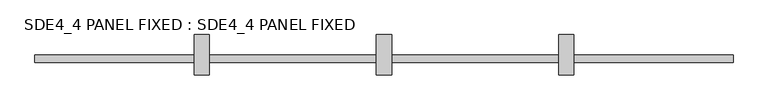
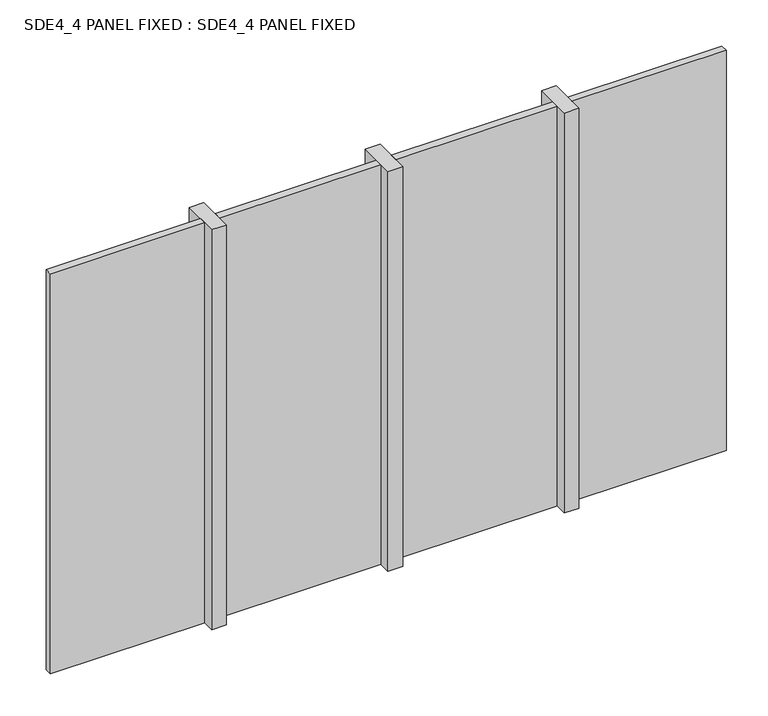
"""IFC4 building model written with IfcOpenShell, lengths in millimetres: plate geometry, SDE4_4 PANEL FIXED : SDE4_4 PANEL FIXED."""

from ifc_helpers import new_model, si_unit, origin, origin_with_axes, place, context, project, spatial, polyline, outline, extrude, source, transform, mapped, element, save


def sde4_4_panel_fixed_sde4_4_panel_fixed_98c40483(model_context):
    return source(origin(), model_context, "Body", "SweptSolid", [
        extrude(outline(polyline([(-1150.0, -132.5), (-1250.0, -132.5), (-1250.0, 132.5), (-1150.0, 132.5), (-1150.0, -132.5)])), origin_with_axes(), (0.0, 0.0, 1.0), 2880.0),
        extrude(outline(polyline([(50.0, -132.5), (-50.0, -132.5), (-50.0, 132.5), (50.0, 132.5), (50.0, -132.5)])), origin_with_axes(), (0.0, 0.0, 1.0), 2880.0),
        extrude(outline(polyline([(1250.0, -132.5), (1150.0, -132.5), (1150.0, 132.5), (1250.0, 132.5), (1250.0, -132.5)])), origin_with_axes(), (0.0, 0.0, 1.0), 2880.0),
        extrude(outline(polyline([(2299.0, -50.0), (1250.0, -50.0), (1250.0, 0.0), (2299.0, 0.0), (2299.0, -50.0)])), origin_with_axes(), (0.0, 0.0, 1.0), 2880.0),
        extrude(outline(polyline([(1150.0, -50.0), (50.0, -50.0), (50.0, 0.0), (1150.0, 0.0), (1150.0, -50.0)])), origin_with_axes(), (0.0, 0.0, 1.0), 2880.0),
        extrude(outline(polyline([(-50.0, -50.0), (-1150.0, -50.0), (-1150.0, 0.0), (-50.0, 0.0), (-50.0, -50.0)])), origin_with_axes(), (0.0, 0.0, 1.0), 2880.0),
        extrude(outline(polyline([(-1250.0, -50.0), (-2300.0, -50.0), (-2300.0, 0.0), (-1250.0, 0.0), (-1250.0, -50.0)])), origin_with_axes(), (0.0, 0.0, 1.0), 2880.0),
    ])


if __name__ == "__main__":
    model = new_model("IFC4")
    model_context = context("Model", 3, world=origin())
    ifc_project = project(units=[si_unit("LENGTHUNIT", "METRE", prefix="MILLI")], contexts=[model_context])
    site = spatial("IfcSite", under=ifc_project)
    building = spatial("IfcBuilding", under=site)
    placement = place(None, origin())
    sde4_4_panel_fixed_sde4_4_panel_fixed_shape = sde4_4_panel_fixed_sde4_4_panel_fixed_98c40483(model_context)
    element("IfcPlate", 1, ObjectType="SDE4_4 PANEL FIXED : SDE4_4 PANEL FIXED", at=placement, inside=building, context=model_context, shape_type="MappedRepresentation", body=[
        mapped(sde4_4_panel_fixed_sde4_4_panel_fixed_shape, transform((0.0, 0.0, 0.0), x_axis=(1.0, 0.0, 0.0), y_axis=(0.0, 1.0, 0.0), z_axis=(0.0, 0.0, 1.0))),
    ])
    save(model, "model.ifc")

# Revit data of these elements
# Type "SDE4_4 PANEL FIXED : SDE4_4 PANEL FIXED"
#   Type Mark = "CW-GLASS"
#   Analytic Construction = "<None>"
#   Glass = Glass
#   Frame = Aluminium
# Element 1 (IfcPlate, "SDE4_4 PANEL FIXED : SDE4_4 PANEL FIXED")
#   Materials on its faces: "Glass", "Aluminium"
# Materials
#   "Glass": class "Glass", colour RGB 0 128 192, transparency 0.9, Keynote = "L40", Cost = 0
#   "Aluminium": class "Unassigned", colour RGB 247 247 247, transparency 0, Cost = 0
